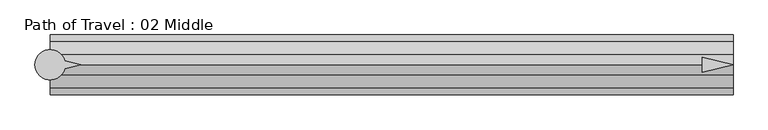
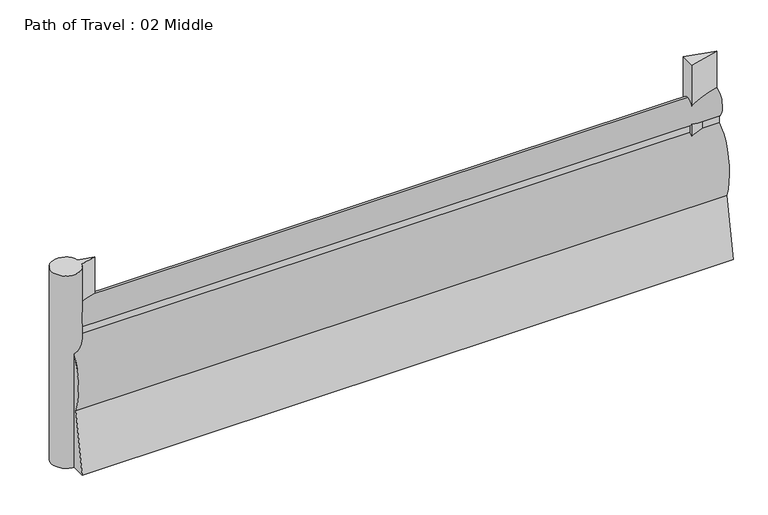
"""IFC4 building model written with IfcOpenShell, lengths in millimetres: proxy geometry, Path of Travel : 02 Middle."""

from ifc_helpers import new_model, si_unit, point, frame, frame_2d, origin, origin_with_axes, place, context, project, spatial, polyline, circle_curve, ellipse_curve, trimmed, segment, composite_curve, outline, extrude, source, transform, mapped, element, save
from ifc_brep_helpers import plane_surface, extruded_surface, advanced_brep


def path_of_travel_02_middle_0f150a4b(model_context):
    return source(origin(), model_context, "Body", "SolidModel", [
        advanced_brep(
        [(227.5554837, 0.0, 1727.2), (227.5554837, 42.9018657, 1436.6534209), (227.5554837, 42.9018657, 1363.4763406), (227.5554837, 184.1186263, 643.4144547), (227.5554837, 297.5699544, 0.0), (227.5554837, 145.6574193, 0.0), (227.5554837, 0.0, 584.2), (227.5554837, -145.6574193, 0.0), (227.5554837, -297.5699544, 0.0), (227.5554837, -184.1186263, 643.4144547), (227.5554837, -42.9018657, 1363.4763406), (227.5554837, -42.9018657, 1436.6534209), (7040.5088187, 0.0, 1727.2), (7040.5088187, -42.9018657, 1436.6534209), (7040.5088187, -42.9018657, 1363.4763406), (7040.5088187, -184.1186263, 643.4144547), (7040.5088187, -297.5699544, 0.0), (7040.5088187, -145.6574193, 0.0), (7040.5088187, 0.0, 584.2), (7040.5088187, 145.6574193, 0.0), (7040.5088187, 297.5699544, 0.0), (7040.5088187, 184.1186263, 643.4144547), (7040.5088187, 42.9018657, 1363.4763406), (7040.5088187, 42.9018657, 1436.6534209)],
        [
            (0, 1, ellipse_curve(frame((227.5554837, 0.0, 1574.8), z_axis=(-1.0, 0.0, 0.0), x_axis=(0.0, 0.0, 1.0)), 152.4, 101.6)),
            (1, 2),
            (2, 3, ellipse_curve(frame((227.5554837, 0.0, 914.4), z_axis=(-1.0, 0.0, 0.0), x_axis=(0.0, 0.0, -1.0)), 457.2, 228.6)),
            (3, 4),
            (4, 5),
            (5, 6),
            (6, 7),
            (7, 8),
            (8, 9),
            (9, 10, ellipse_curve(frame((227.5554837, 0.0, 914.4), z_axis=(-1.0, 0.0, 0.0), x_axis=(0.0, 0.0, -1.0)), 457.2, 228.6)),
            (10, 11),
            (11, 0, ellipse_curve(frame((227.5554837, 0.0, 1574.8), z_axis=(-1.0, 0.0, 0.0), x_axis=(0.0, 0.0, 1.0)), 152.4, 101.6)),
            (12, 13, ellipse_curve(frame((7040.5088187, 0.0, 1574.8), z_axis=(1.0, 0.0, 0.0), x_axis=(0.0, 0.0, 1.0)), 152.4, 101.6)),
            (13, 14),
            (14, 15, ellipse_curve(frame((7040.5088187, 0.0, 914.4), z_axis=(1.0, 0.0, 0.0), x_axis=(0.0, 0.0, -1.0)), 457.2, 228.6)),
            (15, 16),
            (16, 17),
            (17, 18),
            (18, 19),
            (19, 20),
            (20, 21),
            (21, 22, ellipse_curve(frame((7040.5088187, 0.0, 914.4), z_axis=(1.0, 0.0, 0.0), x_axis=(0.0, 0.0, -1.0)), 457.2, 228.6)),
            (22, 23),
            (23, 12, ellipse_curve(frame((7040.5088187, 0.0, 1574.8), z_axis=(1.0, 0.0, 0.0), x_axis=(0.0, 0.0, 1.0)), 152.4, 101.6)),
            (0, 12),
            (23, 1),
            (22, 2),
            (21, 3),
            (20, 4),
            (19, 5),
            (18, 6),
            (17, 7),
            (16, 8),
            (15, 9),
            (14, 10),
            (13, 11),
        ],
        [
            plane_surface(frame((227.5554837, 0.0, 0.0), z_axis=(-1.0, 0.0, 0.0), x_axis=(0.0, 0.0, 1.0))),
            plane_surface(frame((7040.5088187, 0.0, 0.0), z_axis=(1.0, 0.0, 0.0), x_axis=(0.0, 0.0, 1.0))),
            extruded_surface(trimmed(ellipse_curve(frame((7040.5088187, 0.0, 1574.8), z_axis=(-1.0, 0.0, 0.0), x_axis=(0.0, 0.0, 1.0)), 152.4, 101.6), [point((7040.5088187, 0.0, 1727.2))], [point((7040.5088187, 42.9018657, 1436.6534209))], True, "CARTESIAN"), (-6812.953335, 0.0, 0.0), 6812.953335),
            plane_surface(frame((227.5554837, 42.9018657, 1436.6534209), z_axis=(0.0, 1.0, 0.0), x_axis=(1.0, 0.0, 0.0))),
            extruded_surface(trimmed(ellipse_curve(frame((7040.5088187, 0.0, 914.4), z_axis=(-1.0, 0.0, 0.0), x_axis=(0.0, 0.0, -1.0)), 457.2, 228.6), [point((7040.5088187, 42.9018657, 1363.4763406))], [point((7040.5088187, 184.1186263, 643.4144547))], True, "CARTESIAN"), (-6812.953335, 0.0, 0.0), 6812.953335),
            plane_surface(frame((227.5554837, 184.1186263, 643.4144547), z_axis=(0.0, 0.9848077530122078, 0.1736481776669322), x_axis=(1.0, 0.0, 0.0))),
            plane_surface(frame((227.5554837, 297.5699544, 0.0), z_axis=(0.0, 0.0, -1.0), x_axis=(1.0, 0.0, 0.0))),
            plane_surface(frame((227.5554837, 145.6574193, 0.0), z_axis=(0.0, -0.9702957262760199, -0.2419218955995739), x_axis=(1.0, 0.0, 0.0))),
            plane_surface(frame((227.5554837, 0.0, 584.2), z_axis=(0.0, 0.9702957262759961, -0.24192189559966923), x_axis=(1.0, 0.0, 0.0))),
            plane_surface(frame((227.5554837, -145.6574193, 0.0), z_axis=(0.0, 0.0, -1.0), x_axis=(1.0, 0.0, 0.0))),
            plane_surface(frame((227.5554837, -297.5699544, 0.0), z_axis=(0.0, -0.984807753012208, 0.17364817766693066), x_axis=(1.0, 0.0, 0.0))),
            extruded_surface(trimmed(ellipse_curve(frame((7040.5088187, 0.0, 914.4), z_axis=(-1.0, 0.0, 0.0), x_axis=(0.0, 0.0, -1.0)), 457.2, 228.6), [point((7040.5088187, -184.1186263, 643.4144547))], [point((7040.5088187, -42.9018657, 1363.4763406))], True, "CARTESIAN"), (-6812.953335, 0.0, 0.0), 6812.953335),
            plane_surface(frame((227.5554837, -42.9018657, 1363.4763406), z_axis=(0.0, -1.0, 0.0), x_axis=(1.0, 0.0, 0.0))),
            extruded_surface(trimmed(ellipse_curve(frame((7040.5088187, 0.0, 1574.8), z_axis=(-1.0, 0.0, 0.0), x_axis=(0.0, 0.0, 1.0)), 152.4, 101.6), [point((7040.5088187, -42.9018657, 1436.6534209))], [point((7040.5088187, 0.0, 1727.2))], True, "CARTESIAN"), (-6812.953335, 0.0, 0.0), 6812.953335),
        ],
        [
            (0, [[1, 2, 3, 4, 5, 6, 7, 8, 9, 10, 11, 12]]),
            (1, [[13, 14, 15, 16, 17, 18, 19, 20, 21, 22, 23, 24]]),
            (2, [[-1, 25, -24, 26]]),
            (3, [[-2, -26, -23, 27]]),
            (4, [[-3, -27, -22, 28]]),
            (5, [[-4, -28, -21, 29]]),
            (6, [[-5, -29, -20, 30]]),
            (7, [[-6, -30, -19, 31]]),
            (8, [[-7, -31, -18, 32]]),
            (9, [[-8, -32, -17, 33]]),
            (10, [[-9, -33, -16, 34]]),
            (11, [[-10, -34, -15, 35]]),
            (12, [[-11, -35, -14, 36]]),
            (13, [[-12, -36, -13, -25]]),
        ],
    ),
        extrude(outline(polyline([(6734.5036722, 76.2006338), (7040.5088187, 0.0), (6734.5036722, -76.2006338), (6734.5036722, 76.2006338)])), origin_with_axes(), (0.0, 0.0, 1.0), 2129.5973753),
        extrude(outline(composite_curve([segment(polyline([(372.7837828, 39.4440225), (531.182385, 0.0), (372.7837828, -39.4440225)]), True, "CONTINUOUS"), segment(trimmed(circle_curve(frame_2d((227.2200886, 0.0)), 150.8131956), [point((372.7837828, -39.4440225))], [point((372.7837828, 39.4440225))], False, "CARTESIAN"), True, "CONTINUOUS")], self_intersect=False)), origin_with_axes(), (0.0, 0.0, 1.0), 2129.5973753),
    ])


if __name__ == "__main__":
    model = new_model("IFC4")
    model_context = context("Model", 3, world=origin())
    ifc_project = project(units=[si_unit("LENGTHUNIT", "METRE", prefix="MILLI")], contexts=[model_context])
    site = spatial("IfcSite", under=ifc_project)
    building = spatial("IfcBuilding", under=site)
    placement = place(None, origin())
    path_of_travel_02_middle_shape = path_of_travel_02_middle_0f150a4b(model_context)
    element("IfcBuildingElementProxy", 1, Name="Path of Travel : 02 Middle", ObjectType="Path of Travel : 02 Middle", at=placement, inside=building, context=model_context, shape_type="MappedRepresentation", body=[
        mapped(path_of_travel_02_middle_shape, transform((0.0, 0.0, 0.0), x_axis=(1.0, 0.0, 0.0), y_axis=(0.0, 1.0, 0.0), z_axis=(0.0, 0.0, 1.0))),
    ])
    save(model, "model.ifc")

# Revit data of these elements
# Type "Path of Travel : 02 Middle"
#   Path of Egress [instance default] = 4' - 0"
#   built-in parameter 1001306 [instance default] = 4 (stored number, unit not read)
#   Dot at Start = no
#   Arrow in Middle = yes
#   Arrow at End = no
#   Egress Path = none
# Element 1 (IfcBuildingElementProxy, "Path of Travel : 02 Middle")
#   Path of Egress = 22' - 4.22651"
#   built-in parameter 1001306 = 22.3522 (stored number, unit not read)
